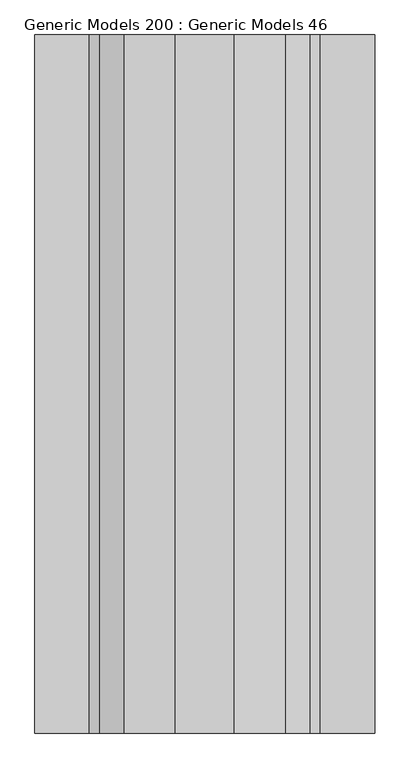
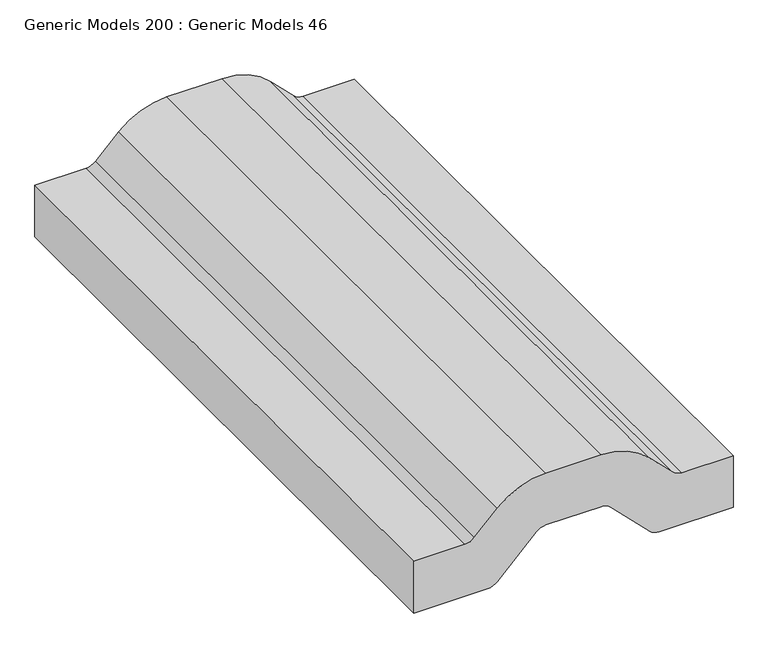
"""IFC4 building model written with IfcOpenShell, lengths in millimetres: proxy geometry, Generic Models 200 : Generic Models 46."""

import ifcopenshell
import ifcopenshell.guid

model = None  # the IFC model being written
_history = None  # IfcOwnerHistory: only IFC2X3 demands one
_inside = {}  # id of a spatial element -> (the spatial element, [elements in it])
_under = {}  # id of a project, library or spatial element -> (it, [spatial elements below it])
_declared = {}  # id of a project -> (the project, [libraries it declares])
_typed = {}  # id of a type object -> (the type object, [elements of that type])
_made_of = {}  # id of a material, layer set ... -> (it, [elements and type objects made of it])


def new_model(schema):
    """Start an empty IFC model of exactly this schema.

    Asked for "IFC4X3", IfcOpenShell would pick the latest addendum, in which some entities
    have other attributes; the version numbers below select the first issue.
    IFC2X3 requires an IfcOwnerHistory on every rooted entity: one is made here for all.
    """
    global model, _history
    if schema == "IFC4X3":
        model = ifcopenshell.file(schema_version=(4, 3, 0, 0))
    else:
        model = ifcopenshell.file(schema=schema)
    _inside.clear()
    _under.clear()
    _declared.clear()
    _typed.clear()
    _made_of.clear()
    _history = None
    if model.schema == "IFC2X3":
        org = make("IfcOrganization", Name="unknown")
        user = make(
            "IfcPersonAndOrganization",
            ThePerson=make("IfcPerson", FamilyName="unknown"),
            TheOrganization=org,
        )
        app = make(
            "IfcApplication",
            ApplicationDeveloper=org,
            Version="unknown",
            ApplicationFullName="unknown",
            ApplicationIdentifier="unknown",
        )
        _history = make(
            "IfcOwnerHistory",
            OwningUser=user,
            OwningApplication=app,
            ChangeAction="ADDED",
            CreationDate=0,
        )
    return model


def make(cls, **values):
    """One entity of the class cls with the attributes given. An attribute that is None is left unset."""
    return model.create_entity(
        cls, **{name: value for name, value in values.items() if value is not None}
    )


def rooted(cls, **values):
    """An entity with a GlobalId (a new one), such as an element, a storey or a relation."""
    return make(cls, GlobalId=ifcopenshell.guid.new(), OwnerHistory=_history, **values)


def si_unit(unit_type, name, prefix=None):
    """IfcSIUnit, for example si_unit("LENGTHUNIT", "METRE", prefix="MILLI")."""
    return make("IfcSIUnit", UnitType=unit_type, Prefix=prefix, Name=name)


def assignment(units):
    """IfcUnitAssignment: the units of a project."""
    return None if units is None else make("IfcUnitAssignment", Units=units)


def point(xyz):
    """IfcCartesianPoint."""
    return None if xyz is None else make("IfcCartesianPoint", Coordinates=xyz)


def direction(xyz):
    """IfcDirection."""
    return None if xyz is None else make("IfcDirection", DirectionRatios=xyz)


def frame(location, z_axis=None, x_axis=None):
    """IfcAxis2Placement3D, a coordinate frame: its origin and axes. An axis left out is left unset."""
    return make(
        "IfcAxis2Placement3D",
        Location=point(location),
        Axis=direction(z_axis),
        RefDirection=direction(x_axis),
    )


def frame_2d(location, x_axis=None):
    """IfcAxis2Placement2D, a coordinate frame in the plane: its origin and x axis."""
    return make(
        "IfcAxis2Placement2D", Location=point(location), RefDirection=direction(x_axis)
    )


def origin():
    """The frame at (0, 0, 0) with its axes left unset."""
    return frame((0.0, 0.0, 0.0))


def place(relative_to, where):
    """IfcLocalPlacement: puts the frame where relative to a parent placement (None: the world)."""
    return make(
        "IfcLocalPlacement", PlacementRelTo=relative_to, RelativePlacement=where
    )


def context(
    kind, dimensions, precision=None, world=None, true_north=None, identifier=None
):
    """IfcGeometricRepresentationContext, for example the 3D "Model" context."""
    return make(
        "IfcGeometricRepresentationContext",
        ContextIdentifier=identifier,
        ContextType=kind,
        CoordinateSpaceDimension=dimensions,
        Precision=precision,
        WorldCoordinateSystem=world,
        TrueNorth=true_north,
    )


def project(units=None, contexts=None):
    """IfcProject with its units and contexts."""
    return rooted(
        "IfcProject",
        Name="project",
        RepresentationContexts=contexts,
        UnitsInContext=assignment(units),
    )


def spatial(cls, under=None, at=None, **own):
    """A site, building, storey or space (cls), placed at a placement, below another one or the project."""
    s = rooted(cls, ObjectPlacement=at, **own)
    if under is not None:
        _under.setdefault(under.id(), (under, []))[1].append(s)
    return s


def polyline(points):
    """IfcPolyline through the points."""
    return make("IfcPolyline", Points=[point(p) for p in points])


def circle_curve(where, radius):
    """IfcCircle in the frame where."""
    return make("IfcCircle", Position=where, Radius=radius)


def trimmed(basis, trim1, trim2, sense, master):
    """IfcTrimmedCurve: the piece of a basis curve between two trims."""
    return make(
        "IfcTrimmedCurve",
        BasisCurve=basis,
        Trim1=trim1,
        Trim2=trim2,
        SenseAgreement=sense,
        MasterRepresentation=master,
    )


def segment(curve, same_sense, transition):
    """IfcCompositeCurveSegment."""
    return make(
        "IfcCompositeCurveSegment",
        Transition=transition,
        SameSense=same_sense,
        ParentCurve=curve,
    )


def composite_curve(segments, self_intersect=None):
    """IfcCompositeCurve: segments joined end to end."""
    return make("IfcCompositeCurve", Segments=segments, SelfIntersect=self_intersect)


def outline(outer, holes=None, kind="AREA"):
    """IfcArbitraryClosedProfileDef: a profile drawn as a closed curve; with holes, ...WithVoids."""
    if holes is None:
        return make("IfcArbitraryClosedProfileDef", ProfileType=kind, OuterCurve=outer)
    return make(
        "IfcArbitraryProfileDefWithVoids",
        ProfileType=kind,
        OuterCurve=outer,
        InnerCurves=holes,
    )


def extrude(swept, where, along, depth):
    """IfcExtrudedAreaSolid: the profile swept, set in the frame where, extruded along a direction by depth."""
    return make(
        "IfcExtrudedAreaSolid",
        SweptArea=swept,
        Position=where,
        ExtrudedDirection=direction(along),
        Depth=depth,
    )


def shape(context_of_items, identifier, shape_type, items):
    """IfcShapeRepresentation: the items that make up one representation, for example the "Body"."""
    return make(
        "IfcShapeRepresentation",
        ContextOfItems=context_of_items,
        RepresentationIdentifier=identifier,
        RepresentationType=shape_type,
        Items=items,
    )


def source(mapping_origin, context_of_items, identifier, shape_type, items):
    """IfcRepresentationMap: a shape defined once, which mapped items show again and again."""
    return make(
        "IfcRepresentationMap",
        MappingOrigin=mapping_origin,
        MappedRepresentation=shape(context_of_items, identifier, shape_type, items),
    )


def transform(
    local_origin,
    x_axis=None,
    y_axis=None,
    z_axis=None,
    scale=None,
    scale2=None,
    scale3=None,
    uniform=True,
):
    """IfcCartesianTransformationOperator3D, or its non-uniform kind. x_axis, y_axis, z_axis: its Axis1, 2, 3."""
    if uniform:
        return make(
            "IfcCartesianTransformationOperator3D",
            Axis1=direction(x_axis),
            Axis2=direction(y_axis),
            LocalOrigin=point(local_origin),
            Scale=scale,
            Axis3=direction(z_axis),
        )
    return make(
        "IfcCartesianTransformationOperator3DnonUniform",
        Axis1=direction(x_axis),
        Axis2=direction(y_axis),
        LocalOrigin=point(local_origin),
        Scale=scale,
        Axis3=direction(z_axis),
        Scale2=scale2,
        Scale3=scale3,
    )


def mapped(mapping_source, mapping_target):
    """IfcMappedItem: shows the shape of a source again, moved by a transform."""
    return make(
        "IfcMappedItem", MappingSource=mapping_source, MappingTarget=mapping_target
    )


def made_of(thing, what):
    """Note that an element or type object is made of a material, layer set ...; save() writes the relation."""
    if what is not None:
        _made_of.setdefault(what.id(), (what, []))[1].append(thing)
    return thing


def element(
    cls,
    number,
    at=None,
    inside=None,
    cuts=None,
    type_object=None,
    material=None,
    context=None,
    identifier="Body",
    shape_type=None,
    held_by="IfcProductDefinitionShape",
    body=None,
    shapes=None,
    **own,
):
    """One element of the class cls, such as IfcWall. Its Tag is "e" and its number.

    at: its placement. inside: the storey or other place that contains it. cuts: it is an
    opening in that element (IfcRelVoidsElement). A single representation is given by context,
    identifier, shape_type and body (its items); several are given by shapes. held_by: the class
    of the entity that holds the representations. save() writes the other relations.
    """
    e = rooted(cls, Tag="e%d" % number, ObjectPlacement=at, **own)
    if body is not None:
        shapes = [shape(context, identifier, shape_type, body)]
    if shapes is not None:
        e.Representation = make(held_by, Representations=shapes)
    if inside is not None:
        _inside.setdefault(inside.id(), (inside, []))[1].append(e)
    if cuts is not None:
        rooted(
            "IfcRelVoidsElement", RelatingBuildingElement=cuts, RelatedOpeningElement=e
        )
    if type_object is not None:
        _typed.setdefault(type_object.id(), (type_object, []))[1].append(e)
    return made_of(e, material)


def aggregate(whole, parts):
    """IfcRelAggregates: a whole, such as a stair, and the parts it consists of."""
    return rooted("IfcRelAggregates", RelatingObject=whole, RelatedObjects=parts)


def save(model, path):
    """Write the relations noted so far, then the file.

    IfcRelAggregates (storeys below a building ...), IfcRelContainedInSpatialStructure (elements
    in a storey), IfcRelDefinesByType, IfcRelAssociatesMaterial and IfcRelDeclares: one each for
    every whole, place, type object, material and project.
    """
    for whole, parts in _under.values():
        aggregate(whole, parts)
    for where, things in _inside.values():
        rooted(
            "IfcRelContainedInSpatialStructure",
            RelatedElements=things,
            RelatingStructure=where,
        )
    for kind, things in _typed.values():
        rooted("IfcRelDefinesByType", RelatedObjects=things, RelatingType=kind)
    for what, things in _made_of.values():
        rooted("IfcRelAssociatesMaterial", RelatedObjects=things, RelatingMaterial=what)
    for by, libraries in _declared.values():
        rooted("IfcRelDeclares", RelatingContext=by, RelatedDefinitions=libraries)
    model.write(path)


def generic_models_200_generic_models_46_d53a038a(model_context):
    return source(origin(), model_context, "Body", "SweptSolid", [
        extrude(outline(composite_curve([segment(trimmed(circle_curve(frame_2d((2162.8204978, 47350.9539755)), 25.4), [point((2188.2204978, 47350.9539755))], [point((2180.7810101, 47368.9144878))], True, "CARTESIAN"), True, "CONTINUOUS"), segment(polyline([(2180.7810101, 47368.9144878), (2108.3699157, 47441.3255821)]), True, "CONTINUOUS"), segment(trimmed(circle_curve(frame_2d((2126.330428, 47459.2860944)), 25.4), [point((2108.3699157, 47441.3255821))], [point((2100.930428, 47459.2860944))], False, "CARTESIAN"), True, "CONTINUOUS"), segment(polyline([(2100.930428, 47459.2860944), (2100.930428, 47596.425), (2202.530428, 47596.425), (2202.530428, 47501.3701923)]), True, "CONTINUOUS"), segment(trimmed(circle_curve(frame_2d((2227.930428, 47501.3701923)), 25.4), [point((2202.530428, 47501.3701923))], [point((2209.9699157, 47483.4096801))], True, "CARTESIAN"), True, "CONTINUOUS"), segment(polyline([(2209.9699157, 47483.4096801), (2252.623059, 47440.7565367)]), True, "CONTINUOUS"), segment(trimmed(circle_curve(frame_2d((2162.8204978, 47350.9539755)), 127.0), [point((2252.623059, 47440.7565367))], [point((2289.8204978, 47350.9539755))], False, "CARTESIAN"), True, "CONTINUOUS"), segment(polyline([(2289.8204978, 47350.9539755), (2289.8204978, 47248.1710245)]), True, "CONTINUOUS"), segment(trimmed(circle_curve(frame_2d((2162.8204978, 47248.1710245)), 127.0), [point((2289.8204978, 47248.1710245))], [point((2252.623059, 47158.3684633))], False, "CARTESIAN"), True, "CONTINUOUS"), segment(polyline([(2252.623059, 47158.3684633), (2209.9699157, 47115.7153199)]), True, "CONTINUOUS"), segment(trimmed(circle_curve(frame_2d((2227.930428, 47097.7548077)), 25.4), [point((2209.9699157, 47115.7153199))], [point((2202.530428, 47097.7548077))], True, "CARTESIAN"), True, "CONTINUOUS"), segment(polyline([(2202.530428, 47097.7548077), (2202.530428, 47002.7), (2100.930428, 47002.7), (2100.930428, 47139.8389056)]), True, "CONTINUOUS"), segment(trimmed(circle_curve(frame_2d((2126.330428, 47139.8389056)), 25.4), [point((2100.930428, 47139.8389056))], [point((2108.3699157, 47157.7994179))], False, "CARTESIAN"), True, "CONTINUOUS"), segment(polyline([(2108.3699157, 47157.7994179), (2180.7810101, 47230.2105122)]), True, "CONTINUOUS"), segment(trimmed(circle_curve(frame_2d((2162.8204978, 47248.1710245)), 25.4), [point((2180.7810101, 47230.2105122))], [point((2188.2204978, 47248.1710245))], True, "CARTESIAN"), True, "CONTINUOUS"), segment(polyline([(2188.2204978, 47248.1710245), (2188.2204978, 47350.9539755)]), True, "CONTINUOUS")], self_intersect=False)), frame((0.0, 0.0, 0.0), z_axis=(0.0, 1.0, 0.0), x_axis=(0.0, 0.0, 1.0)), (0.0, 0.0, 1.0), 1219.2),
    ])


if __name__ == "__main__":
    model = new_model("IFC4")
    model_context = context("Model", 3, world=origin())
    ifc_project = project(units=[si_unit("LENGTHUNIT", "METRE", prefix="MILLI")], contexts=[model_context])
    site = spatial("IfcSite", under=ifc_project)
    building = spatial("IfcBuilding", under=site)
    placement = place(None, origin())
    generic_models_200_generic_models_46_shape = generic_models_200_generic_models_46_d53a038a(model_context)
    element("IfcBuildingElementProxy", 1, Name="Generic Models 200 : Generic Models 46", ObjectType="Generic Models 200 : Generic Models 46", at=placement, inside=building, context=model_context, shape_type="MappedRepresentation", body=[
        mapped(generic_models_200_generic_models_46_shape, transform((0.0, 0.0, 0.0), x_axis=(1.0, 0.0, 0.0), y_axis=(0.0, 1.0, 0.0), z_axis=(0.0, 0.0, 1.0))),
    ])
    save(model, "model.ifc")

# Revit data of these elements
# Element 1 (IfcBuildingElementProxy, "Generic Models 200 : Generic Models 46")
#   Materials on its faces: "BATT. INSULATION - EXTEND 4'-0\" MIN. - EACH SIDE OF STUD"
# Materials
#   "BATT. INSULATION - EXTEND 4'-0\" MIN. - EACH SIDE OF STUD": class "Unassigned", colour RGB 255 255 255, transparency 0, Cost = 0
